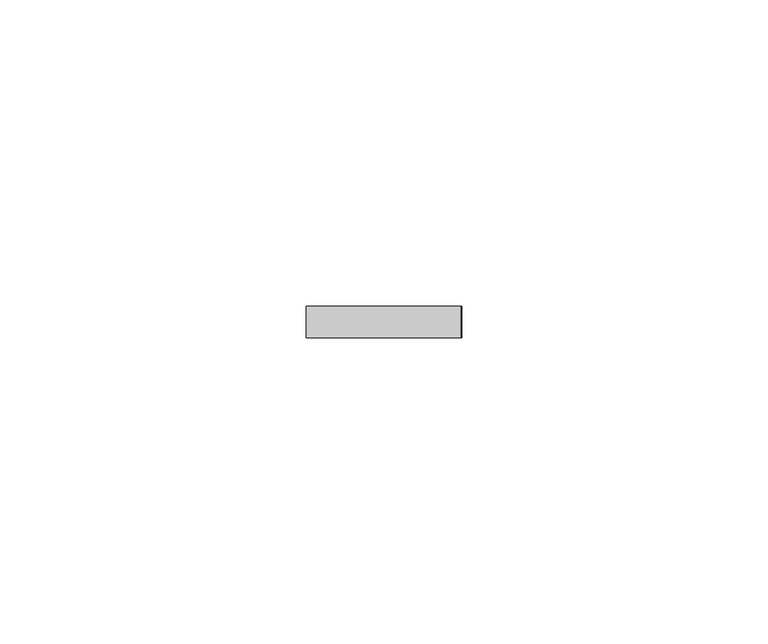
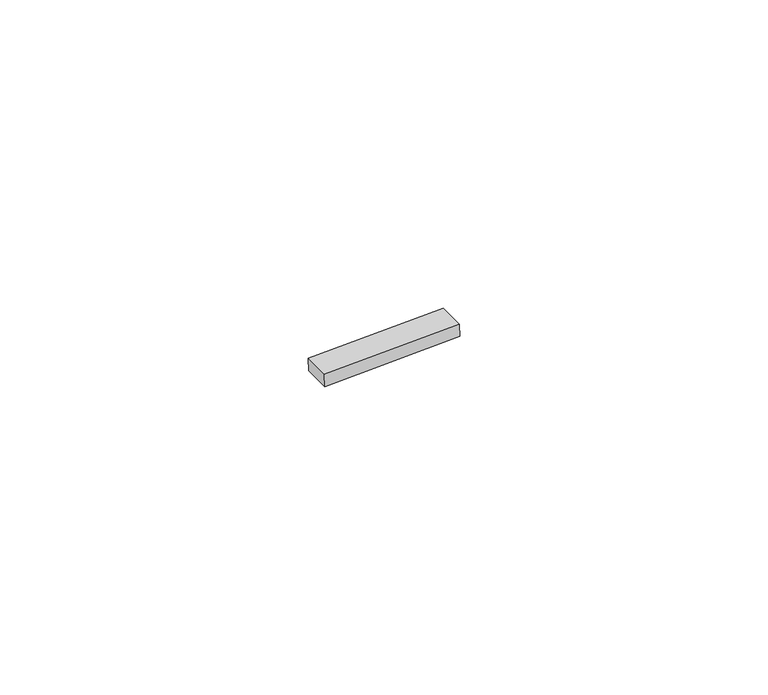
"""IFC4 building model written with IfcOpenShell, lengths in millimetres: proxy geometry, Inner panel:Inner panel:1:Inner panel:1 : Inner panel:Inner panel:300324:2:Inner panel:1:Inner panel:1 : Inner panel:Inner panel:300324:2 : Inner panel:Inner panel:1:Inner panel:1 : Inner panel:Inner panel:300324:300043:151 : Inner panel:Inner panel:1:Inner panel:1 : Inner panel:Inner panel:300324:2:Inner panel:1:Inner panel:1 : Inner panel:Inner panel:300324:2 : Inner panel:Inner panel:1:Inner panel:1 : Inner panel:Inner panel:300324:300043:308120."""

import ifcopenshell
import ifcopenshell.guid

model = None  # the IFC model being written
_history = None  # IfcOwnerHistory: only IFC2X3 demands one
_inside = {}  # id of a spatial element -> (the spatial element, [elements in it])
_under = {}  # id of a project, library or spatial element -> (it, [spatial elements below it])
_declared = {}  # id of a project -> (the project, [libraries it declares])
_typed = {}  # id of a type object -> (the type object, [elements of that type])
_made_of = {}  # id of a material, layer set ... -> (it, [elements and type objects made of it])


def new_model(schema):
    """Start an empty IFC model of exactly this schema.

    Asked for "IFC4X3", IfcOpenShell would pick the latest addendum, in which some entities
    have other attributes; the version numbers below select the first issue.
    IFC2X3 requires an IfcOwnerHistory on every rooted entity: one is made here for all.
    """
    global model, _history
    if schema == "IFC4X3":
        model = ifcopenshell.file(schema_version=(4, 3, 0, 0))
    else:
        model = ifcopenshell.file(schema=schema)
    _inside.clear()
    _under.clear()
    _declared.clear()
    _typed.clear()
    _made_of.clear()
    _history = None
    if model.schema == "IFC2X3":
        org = make("IfcOrganization", Name="unknown")
        user = make(
            "IfcPersonAndOrganization",
            ThePerson=make("IfcPerson", FamilyName="unknown"),
            TheOrganization=org,
        )
        app = make(
            "IfcApplication",
            ApplicationDeveloper=org,
            Version="unknown",
            ApplicationFullName="unknown",
            ApplicationIdentifier="unknown",
        )
        _history = make(
            "IfcOwnerHistory",
            OwningUser=user,
            OwningApplication=app,
            ChangeAction="ADDED",
            CreationDate=0,
        )
    return model


def make(cls, **values):
    """One entity of the class cls with the attributes given. An attribute that is None is left unset."""
    return model.create_entity(
        cls, **{name: value for name, value in values.items() if value is not None}
    )


def rooted(cls, **values):
    """An entity with a GlobalId (a new one), such as an element, a storey or a relation."""
    return make(cls, GlobalId=ifcopenshell.guid.new(), OwnerHistory=_history, **values)


def si_unit(unit_type, name, prefix=None):
    """IfcSIUnit, for example si_unit("LENGTHUNIT", "METRE", prefix="MILLI")."""
    return make("IfcSIUnit", UnitType=unit_type, Prefix=prefix, Name=name)


def assignment(units):
    """IfcUnitAssignment: the units of a project."""
    return None if units is None else make("IfcUnitAssignment", Units=units)


def point(xyz):
    """IfcCartesianPoint."""
    return None if xyz is None else make("IfcCartesianPoint", Coordinates=xyz)


def direction(xyz):
    """IfcDirection."""
    return None if xyz is None else make("IfcDirection", DirectionRatios=xyz)


def frame(location, z_axis=None, x_axis=None):
    """IfcAxis2Placement3D, a coordinate frame: its origin and axes. An axis left out is left unset."""
    return make(
        "IfcAxis2Placement3D",
        Location=point(location),
        Axis=direction(z_axis),
        RefDirection=direction(x_axis),
    )


def origin():
    """The frame at (0, 0, 0) with its axes left unset."""
    return frame((0.0, 0.0, 0.0))


def place(relative_to, where):
    """IfcLocalPlacement: puts the frame where relative to a parent placement (None: the world)."""
    return make(
        "IfcLocalPlacement", PlacementRelTo=relative_to, RelativePlacement=where
    )


def context(
    kind, dimensions, precision=None, world=None, true_north=None, identifier=None
):
    """IfcGeometricRepresentationContext, for example the 3D "Model" context."""
    return make(
        "IfcGeometricRepresentationContext",
        ContextIdentifier=identifier,
        ContextType=kind,
        CoordinateSpaceDimension=dimensions,
        Precision=precision,
        WorldCoordinateSystem=world,
        TrueNorth=true_north,
    )


def project(units=None, contexts=None):
    """IfcProject with its units and contexts."""
    return rooted(
        "IfcProject",
        Name="project",
        RepresentationContexts=contexts,
        UnitsInContext=assignment(units),
    )


def spatial(cls, under=None, at=None, **own):
    """A site, building, storey or space (cls), placed at a placement, below another one or the project."""
    s = rooted(cls, ObjectPlacement=at, **own)
    if under is not None:
        _under.setdefault(under.id(), (under, []))[1].append(s)
    return s


def polyline(points):
    """IfcPolyline through the points."""
    return make("IfcPolyline", Points=[point(p) for p in points])


def outline(outer, holes=None, kind="AREA"):
    """IfcArbitraryClosedProfileDef: a profile drawn as a closed curve; with holes, ...WithVoids."""
    if holes is None:
        return make("IfcArbitraryClosedProfileDef", ProfileType=kind, OuterCurve=outer)
    return make(
        "IfcArbitraryProfileDefWithVoids",
        ProfileType=kind,
        OuterCurve=outer,
        InnerCurves=holes,
    )


def extrude(swept, where, along, depth):
    """IfcExtrudedAreaSolid: the profile swept, set in the frame where, extruded along a direction by depth."""
    return make(
        "IfcExtrudedAreaSolid",
        SweptArea=swept,
        Position=where,
        ExtrudedDirection=direction(along),
        Depth=depth,
    )


def shape(context_of_items, identifier, shape_type, items):
    """IfcShapeRepresentation: the items that make up one representation, for example the "Body"."""
    return make(
        "IfcShapeRepresentation",
        ContextOfItems=context_of_items,
        RepresentationIdentifier=identifier,
        RepresentationType=shape_type,
        Items=items,
    )


def source(mapping_origin, context_of_items, identifier, shape_type, items):
    """IfcRepresentationMap: a shape defined once, which mapped items show again and again."""
    return make(
        "IfcRepresentationMap",
        MappingOrigin=mapping_origin,
        MappedRepresentation=shape(context_of_items, identifier, shape_type, items),
    )


def transform(
    local_origin,
    x_axis=None,
    y_axis=None,
    z_axis=None,
    scale=None,
    scale2=None,
    scale3=None,
    uniform=True,
):
    """IfcCartesianTransformationOperator3D, or its non-uniform kind. x_axis, y_axis, z_axis: its Axis1, 2, 3."""
    if uniform:
        return make(
            "IfcCartesianTransformationOperator3D",
            Axis1=direction(x_axis),
            Axis2=direction(y_axis),
            LocalOrigin=point(local_origin),
            Scale=scale,
            Axis3=direction(z_axis),
        )
    return make(
        "IfcCartesianTransformationOperator3DnonUniform",
        Axis1=direction(x_axis),
        Axis2=direction(y_axis),
        LocalOrigin=point(local_origin),
        Scale=scale,
        Axis3=direction(z_axis),
        Scale2=scale2,
        Scale3=scale3,
    )


def mapped(mapping_source, mapping_target):
    """IfcMappedItem: shows the shape of a source again, moved by a transform."""
    return make(
        "IfcMappedItem", MappingSource=mapping_source, MappingTarget=mapping_target
    )


def made_of(thing, what):
    """Note that an element or type object is made of a material, layer set ...; save() writes the relation."""
    if what is not None:
        _made_of.setdefault(what.id(), (what, []))[1].append(thing)
    return thing


def element(
    cls,
    number,
    at=None,
    inside=None,
    cuts=None,
    type_object=None,
    material=None,
    context=None,
    identifier="Body",
    shape_type=None,
    held_by="IfcProductDefinitionShape",
    body=None,
    shapes=None,
    **own,
):
    """One element of the class cls, such as IfcWall. Its Tag is "e" and its number.

    at: its placement. inside: the storey or other place that contains it. cuts: it is an
    opening in that element (IfcRelVoidsElement). A single representation is given by context,
    identifier, shape_type and body (its items); several are given by shapes. held_by: the class
    of the entity that holds the representations. save() writes the other relations.
    """
    e = rooted(cls, Tag="e%d" % number, ObjectPlacement=at, **own)
    if body is not None:
        shapes = [shape(context, identifier, shape_type, body)]
    if shapes is not None:
        e.Representation = make(held_by, Representations=shapes)
    if inside is not None:
        _inside.setdefault(inside.id(), (inside, []))[1].append(e)
    if cuts is not None:
        rooted(
            "IfcRelVoidsElement", RelatingBuildingElement=cuts, RelatedOpeningElement=e
        )
    if type_object is not None:
        _typed.setdefault(type_object.id(), (type_object, []))[1].append(e)
    return made_of(e, material)


def aggregate(whole, parts):
    """IfcRelAggregates: a whole, such as a stair, and the parts it consists of."""
    return rooted("IfcRelAggregates", RelatingObject=whole, RelatedObjects=parts)


def save(model, path):
    """Write the relations noted so far, then the file.

    IfcRelAggregates (storeys below a building ...), IfcRelContainedInSpatialStructure (elements
    in a storey), IfcRelDefinesByType, IfcRelAssociatesMaterial and IfcRelDeclares: one each for
    every whole, place, type object, material and project.
    """
    for whole, parts in _under.values():
        aggregate(whole, parts)
    for where, things in _inside.values():
        rooted(
            "IfcRelContainedInSpatialStructure",
            RelatedElements=things,
            RelatingStructure=where,
        )
    for kind, things in _typed.values():
        rooted("IfcRelDefinesByType", RelatedObjects=things, RelatingType=kind)
    for what, things in _made_of.values():
        rooted("IfcRelAssociatesMaterial", RelatedObjects=things, RelatingMaterial=what)
    for by, libraries in _declared.values():
        rooted("IfcRelDeclares", RelatingContext=by, RelatedDefinitions=libraries)
    model.write(path)


def generic_models_16917ee4(model_context):
    return source(origin(), model_context, "Body", "SweptSolid", [
        extrude(outline(polyline([(0.0, -25.4), (0.0, 0.0), (5.2138089, 0.0), (5.2138089, -25.4), (0.0, -25.4)])), frame((560380.9331581, -578534.9848948, 3950.5346611), z_axis=(-0.041630544712223896, 0.0, 0.9991330730923502), x_axis=(0.0, -1.0, 0.0)), (0.0, 0.0, 1.0), 2.4763745),
    ])


if __name__ == "__main__":
    model = new_model("IFC4")
    model_context = context("Model", 3, world=origin())
    ifc_project = project(units=[si_unit("LENGTHUNIT", "METRE", prefix="MILLI")], contexts=[model_context])
    site = spatial("IfcSite", under=ifc_project)
    building = spatial("IfcBuilding", under=site)
    placement = place(None, origin())
    generic_models_shape = generic_models_16917ee4(model_context)
    element("IfcBuildingElementProxy", 1, Name="Inner panel:Inner panel:1:Inner panel:1 : Inner panel:Inner panel:300324:2:Inner panel:1:Inner panel:1 : Inner panel:Inner panel:300324:2 : Inner panel:Inner panel:1:Inner panel:1 : Inner panel:Inner panel:300324:300043:151 : Inner panel:Inner panel:1:Inner panel:1 : Inner panel:Inner panel:300324:2:Inner panel:1:Inner panel:1 : Inner panel:Inner panel:300324:2 : Inner panel:Inner panel:1:Inner panel:1 : Inner panel:Inner panel:300324:300043:308120", ObjectType="Inner panel:Inner panel:1:Inner panel:1 : Inner panel:Inner panel:300324:2:Inner panel:1:Inner panel:1 : Inner panel:Inner panel:300324:2 : Inner panel:Inner panel:1:Inner panel:1 : Inner panel:Inner panel:300324:300043:151 : Inner panel:Inner panel:1:Inner panel:1 : Inner panel:Inner panel:300324:2:Inner panel:1:Inner panel:1 : Inner panel:Inner panel:300324:2 : Inner panel:Inner panel:1:Inner panel:1 : Inner panel:Inner panel:300324:300043:308120", at=placement, inside=building, context=model_context, shape_type="MappedRepresentation", body=[
        mapped(generic_models_shape, transform((0.0, 0.0, 0.0), x_axis=(1.0, 0.0, 0.0), y_axis=(0.0, 1.0, 0.0), z_axis=(0.0, 0.0, 1.0))),
    ])
    save(model, "model.ifc")

# Revit data of these elements
# Type "Inner panel:Inner panel:1:Inner panel:1 : Inner panel:Inner panel:300324:2:Inner panel:1:Inner panel:1 : Inner panel:Inner panel:300324:2 : Inner panel:Inner panel:1:Inner panel:1 : Inner panel:Inner panel:300324:300043:151 : Inner panel:Inner panel:1:Inner panel:1 : Inner panel:Inner panel:300324:2:Inner panel:1:Inner panel:1 : Inner panel:Inner panel:300324:2 : Inner panel:Inner panel:1:Inner panel:1 : Inner panel:Inner panel:300324:300043:308120"
#   NameOverride = "Inner panel:Inner panel:1:Inner panel:1 : Inner panel:Inner panel:300324:2:Inner panel:1:Inner panel:1 : Inner panel:Inner panel:300324:2 : Inner panel:Inner panel:1:Inner panel:1 : Inner panel:Inner panel:300324:300043:308120"
#   ObjectTypeOverride = "Inner panel:1:Inner panel:1 : Inner panel:Inner panel:300324:2 : Inner panel:Inner panel:1:Inner panel:1 : Inner panel:Inner panel:300324:300043"
#   Reference = "Inner panel"
#   Tag = "308120"
# Element 1 (IfcBuildingElementProxy, "Inner panel:Inner panel:1:Inner panel:1 : Inner panel:Inner panel:300324:2:Inner panel:1:Inner panel:1 : Inner panel:Inner panel:300324:2 : Inner panel:Inner panel:1:Inner panel:1 : Inner panel:Inner panel:300324:300043:151 : Inner panel:Inner panel:1:Inner panel:1 : Inner panel:Inner panel:300324:2:Inner panel:1:Inner panel:1 : Inner panel:Inner panel:300324:2 : Inner panel:Inner panel:1:Inner panel:1 : Inner panel:Inner panel:300324:300043:308120")
#   Materials on its faces: "AT CLIP - 1\" WIDE NON ABSORBENT, WEATHER-RESISTANT NEOPRENE/EPDM/SBR FOAM"
# Materials
#   "AT CLIP - 1\" WIDE NON ABSORBENT, WEATHER-RESISTANT NEOPRENE/EPDM/SBR FOAM": class "Generic", colour RGB 85 85 85, transparency 0, Cost = 0
